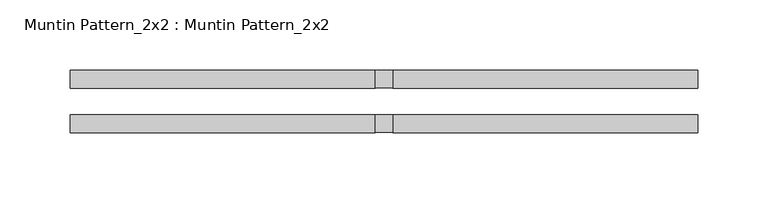
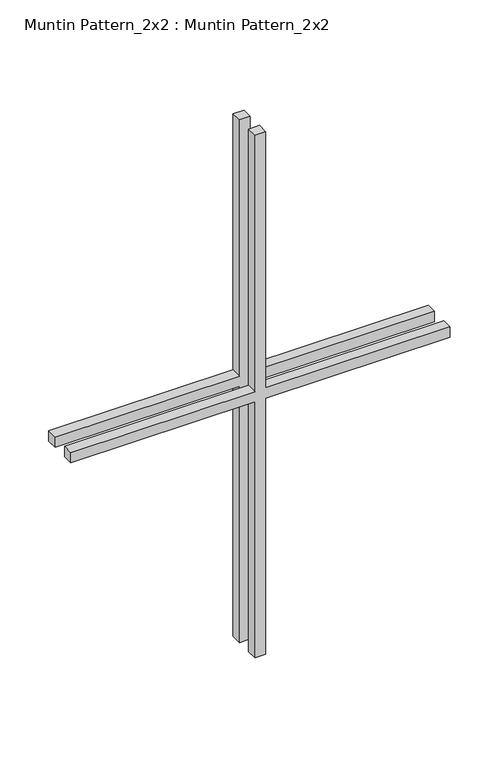
"""IFC4 building model written with IfcOpenShell, lengths in millimetres: proxy geometry, Muntin Pattern_2x2 : Muntin Pattern_2x2."""

import ifcopenshell
import ifcopenshell.guid

model = None  # the IFC model being written
_history = None  # IfcOwnerHistory: only IFC2X3 demands one
_inside = {}  # id of a spatial element -> (the spatial element, [elements in it])
_under = {}  # id of a project, library or spatial element -> (it, [spatial elements below it])
_declared = {}  # id of a project -> (the project, [libraries it declares])
_typed = {}  # id of a type object -> (the type object, [elements of that type])
_made_of = {}  # id of a material, layer set ... -> (it, [elements and type objects made of it])


def new_model(schema):
    """Start an empty IFC model of exactly this schema.

    Asked for "IFC4X3", IfcOpenShell would pick the latest addendum, in which some entities
    have other attributes; the version numbers below select the first issue.
    IFC2X3 requires an IfcOwnerHistory on every rooted entity: one is made here for all.
    """
    global model, _history
    if schema == "IFC4X3":
        model = ifcopenshell.file(schema_version=(4, 3, 0, 0))
    else:
        model = ifcopenshell.file(schema=schema)
    _inside.clear()
    _under.clear()
    _declared.clear()
    _typed.clear()
    _made_of.clear()
    _history = None
    if model.schema == "IFC2X3":
        org = make("IfcOrganization", Name="unknown")
        user = make(
            "IfcPersonAndOrganization",
            ThePerson=make("IfcPerson", FamilyName="unknown"),
            TheOrganization=org,
        )
        app = make(
            "IfcApplication",
            ApplicationDeveloper=org,
            Version="unknown",
            ApplicationFullName="unknown",
            ApplicationIdentifier="unknown",
        )
        _history = make(
            "IfcOwnerHistory",
            OwningUser=user,
            OwningApplication=app,
            ChangeAction="ADDED",
            CreationDate=0,
        )
    return model


def make(cls, **values):
    """One entity of the class cls with the attributes given. An attribute that is None is left unset."""
    return model.create_entity(
        cls, **{name: value for name, value in values.items() if value is not None}
    )


def rooted(cls, **values):
    """An entity with a GlobalId (a new one), such as an element, a storey or a relation."""
    return make(cls, GlobalId=ifcopenshell.guid.new(), OwnerHistory=_history, **values)


def si_unit(unit_type, name, prefix=None):
    """IfcSIUnit, for example si_unit("LENGTHUNIT", "METRE", prefix="MILLI")."""
    return make("IfcSIUnit", UnitType=unit_type, Prefix=prefix, Name=name)


def assignment(units):
    """IfcUnitAssignment: the units of a project."""
    return None if units is None else make("IfcUnitAssignment", Units=units)


def point(xyz):
    """IfcCartesianPoint."""
    return None if xyz is None else make("IfcCartesianPoint", Coordinates=xyz)


def direction(xyz):
    """IfcDirection."""
    return None if xyz is None else make("IfcDirection", DirectionRatios=xyz)


def frame(location, z_axis=None, x_axis=None):
    """IfcAxis2Placement3D, a coordinate frame: its origin and axes. An axis left out is left unset."""
    return make(
        "IfcAxis2Placement3D",
        Location=point(location),
        Axis=direction(z_axis),
        RefDirection=direction(x_axis),
    )


def origin():
    """The frame at (0, 0, 0) with its axes left unset."""
    return frame((0.0, 0.0, 0.0))


def place(relative_to, where):
    """IfcLocalPlacement: puts the frame where relative to a parent placement (None: the world)."""
    return make(
        "IfcLocalPlacement", PlacementRelTo=relative_to, RelativePlacement=where
    )


def context(
    kind, dimensions, precision=None, world=None, true_north=None, identifier=None
):
    """IfcGeometricRepresentationContext, for example the 3D "Model" context."""
    return make(
        "IfcGeometricRepresentationContext",
        ContextIdentifier=identifier,
        ContextType=kind,
        CoordinateSpaceDimension=dimensions,
        Precision=precision,
        WorldCoordinateSystem=world,
        TrueNorth=true_north,
    )


def project(units=None, contexts=None):
    """IfcProject with its units and contexts."""
    return rooted(
        "IfcProject",
        Name="project",
        RepresentationContexts=contexts,
        UnitsInContext=assignment(units),
    )


def spatial(cls, under=None, at=None, **own):
    """A site, building, storey or space (cls), placed at a placement, below another one or the project."""
    s = rooted(cls, ObjectPlacement=at, **own)
    if under is not None:
        _under.setdefault(under.id(), (under, []))[1].append(s)
    return s


def polyline(points):
    """IfcPolyline through the points."""
    return make("IfcPolyline", Points=[point(p) for p in points])


def outline(outer, holes=None, kind="AREA"):
    """IfcArbitraryClosedProfileDef: a profile drawn as a closed curve; with holes, ...WithVoids."""
    if holes is None:
        return make("IfcArbitraryClosedProfileDef", ProfileType=kind, OuterCurve=outer)
    return make(
        "IfcArbitraryProfileDefWithVoids",
        ProfileType=kind,
        OuterCurve=outer,
        InnerCurves=holes,
    )


def extrude(swept, where, along, depth):
    """IfcExtrudedAreaSolid: the profile swept, set in the frame where, extruded along a direction by depth."""
    return make(
        "IfcExtrudedAreaSolid",
        SweptArea=swept,
        Position=where,
        ExtrudedDirection=direction(along),
        Depth=depth,
    )


def shape(context_of_items, identifier, shape_type, items):
    """IfcShapeRepresentation: the items that make up one representation, for example the "Body"."""
    return make(
        "IfcShapeRepresentation",
        ContextOfItems=context_of_items,
        RepresentationIdentifier=identifier,
        RepresentationType=shape_type,
        Items=items,
    )


def source(mapping_origin, context_of_items, identifier, shape_type, items):
    """IfcRepresentationMap: a shape defined once, which mapped items show again and again."""
    return make(
        "IfcRepresentationMap",
        MappingOrigin=mapping_origin,
        MappedRepresentation=shape(context_of_items, identifier, shape_type, items),
    )


def transform(
    local_origin,
    x_axis=None,
    y_axis=None,
    z_axis=None,
    scale=None,
    scale2=None,
    scale3=None,
    uniform=True,
):
    """IfcCartesianTransformationOperator3D, or its non-uniform kind. x_axis, y_axis, z_axis: its Axis1, 2, 3."""
    if uniform:
        return make(
            "IfcCartesianTransformationOperator3D",
            Axis1=direction(x_axis),
            Axis2=direction(y_axis),
            LocalOrigin=point(local_origin),
            Scale=scale,
            Axis3=direction(z_axis),
        )
    return make(
        "IfcCartesianTransformationOperator3DnonUniform",
        Axis1=direction(x_axis),
        Axis2=direction(y_axis),
        LocalOrigin=point(local_origin),
        Scale=scale,
        Axis3=direction(z_axis),
        Scale2=scale2,
        Scale3=scale3,
    )


def mapped(mapping_source, mapping_target):
    """IfcMappedItem: shows the shape of a source again, moved by a transform."""
    return make(
        "IfcMappedItem", MappingSource=mapping_source, MappingTarget=mapping_target
    )


def made_of(thing, what):
    """Note that an element or type object is made of a material, layer set ...; save() writes the relation."""
    if what is not None:
        _made_of.setdefault(what.id(), (what, []))[1].append(thing)
    return thing


def element(
    cls,
    number,
    at=None,
    inside=None,
    cuts=None,
    type_object=None,
    material=None,
    context=None,
    identifier="Body",
    shape_type=None,
    held_by="IfcProductDefinitionShape",
    body=None,
    shapes=None,
    **own,
):
    """One element of the class cls, such as IfcWall. Its Tag is "e" and its number.

    at: its placement. inside: the storey or other place that contains it. cuts: it is an
    opening in that element (IfcRelVoidsElement). A single representation is given by context,
    identifier, shape_type and body (its items); several are given by shapes. held_by: the class
    of the entity that holds the representations. save() writes the other relations.
    """
    e = rooted(cls, Tag="e%d" % number, ObjectPlacement=at, **own)
    if body is not None:
        shapes = [shape(context, identifier, shape_type, body)]
    if shapes is not None:
        e.Representation = make(held_by, Representations=shapes)
    if inside is not None:
        _inside.setdefault(inside.id(), (inside, []))[1].append(e)
    if cuts is not None:
        rooted(
            "IfcRelVoidsElement", RelatingBuildingElement=cuts, RelatedOpeningElement=e
        )
    if type_object is not None:
        _typed.setdefault(type_object.id(), (type_object, []))[1].append(e)
    return made_of(e, material)


def aggregate(whole, parts):
    """IfcRelAggregates: a whole, such as a stair, and the parts it consists of."""
    return rooted("IfcRelAggregates", RelatingObject=whole, RelatedObjects=parts)


def save(model, path):
    """Write the relations noted so far, then the file.

    IfcRelAggregates (storeys below a building ...), IfcRelContainedInSpatialStructure (elements
    in a storey), IfcRelDefinesByType, IfcRelAssociatesMaterial and IfcRelDeclares: one each for
    every whole, place, type object, material and project.
    """
    for whole, parts in _under.values():
        aggregate(whole, parts)
    for where, things in _inside.values():
        rooted(
            "IfcRelContainedInSpatialStructure",
            RelatedElements=things,
            RelatingStructure=where,
        )
    for kind, things in _typed.values():
        rooted("IfcRelDefinesByType", RelatedObjects=things, RelatingType=kind)
    for what, things in _made_of.values():
        rooted("IfcRelAssociatesMaterial", RelatedObjects=things, RelatingMaterial=what)
    for by, libraries in _declared.values():
        rooted("IfcRelDeclares", RelatingContext=by, RelatedDefinitions=libraries)
    model.write(path)


def muntin_pattern_2x2_muntin_pattern_2x2_5bc09aa8(model_context):
    return source(origin(), model_context, "Body", "SweptSolid", [
        extrude(outline(polyline([(332.1375, -6.35), (332.1375, -223.8), (319.4375, -223.8), (319.4375, -6.35), (0.0, -6.35), (0.0, 6.35), (319.4375, 6.35), (319.4375, 223.8), (332.1375, 223.8), (332.1375, 6.35), (651.575, 6.35), (651.575, -6.35), (332.1375, -6.35)])), frame((0.0, 9.525, 0.0), z_axis=(0.0, 1.0, 0.0), x_axis=(0.0, 0.0, 1.0)), (0.0, 0.0, 1.0), 12.7),
        extrude(outline(polyline([(332.1375, -6.35), (332.1375, -223.8), (319.4375, -223.8), (319.4375, -6.35), (0.0, -6.35), (0.0, 6.35), (319.4375, 6.35), (319.4375, 223.8), (332.1375, 223.8), (332.1375, 6.35), (651.575, 6.35), (651.575, -6.35), (332.1375, -6.35)])), frame((0.0, -22.225, 0.0), z_axis=(0.0, 1.0, 0.0), x_axis=(0.0, 0.0, 1.0)), (0.0, 0.0, 1.0), 12.7),
    ])


if __name__ == "__main__":
    model = new_model("IFC4")
    model_context = context("Model", 3, world=origin())
    ifc_project = project(units=[si_unit("LENGTHUNIT", "METRE", prefix="MILLI")], contexts=[model_context])
    site = spatial("IfcSite", under=ifc_project)
    building = spatial("IfcBuilding", under=site)
    placement = place(None, origin())
    muntin_pattern_2x2_muntin_pattern_2x2_shape = muntin_pattern_2x2_muntin_pattern_2x2_5bc09aa8(model_context)
    element("IfcBuildingElementProxy", 1, Name="Muntin Pattern_2x2 : Muntin Pattern_2x2", ObjectType="Muntin Pattern_2x2 : Muntin Pattern_2x2", at=placement, inside=building, context=model_context, shape_type="MappedRepresentation", body=[
        mapped(muntin_pattern_2x2_muntin_pattern_2x2_shape, transform((0.0, 0.0, 0.0), x_axis=(1.0, 0.0, 0.0), y_axis=(0.0, 1.0, 0.0), z_axis=(0.0, 0.0, 1.0))),
    ])
    save(model, "model.ifc")

# Revit data of these elements
# Type "Muntin Pattern_2x2 : Muntin Pattern_2x2"
#   Width [instance default] = 121.92 cm
#   Thickness = 1.27 cm
#   Height [instance default] = 121.92 cm
#   Distance = 1.905 cm
#   Interior Material [instance default] = none
#   Exterior Material [instance default] = none
# Element 1 (IfcBuildingElementProxy, "Muntin Pattern_2x2 : Muntin Pattern_2x2")
#   Width = 44.76 cm
#   Height = 65.1575 cm
#   Interior Material = Wood - Stained
#   Exterior Material = Clad - White
#   Materials on its faces: "Clad - White", "Wood - Stained"
# Materials
#   "Clad - White": class "Wood", colour RGB 242 242 238, transparency 0, Cost = 0
#   "Wood - Stained": class "Wood", colour RGB 224 178 126, transparency 0, Cost = 0
